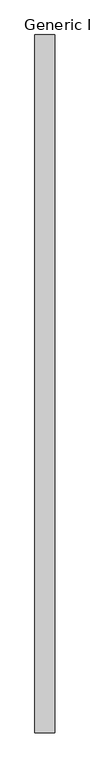
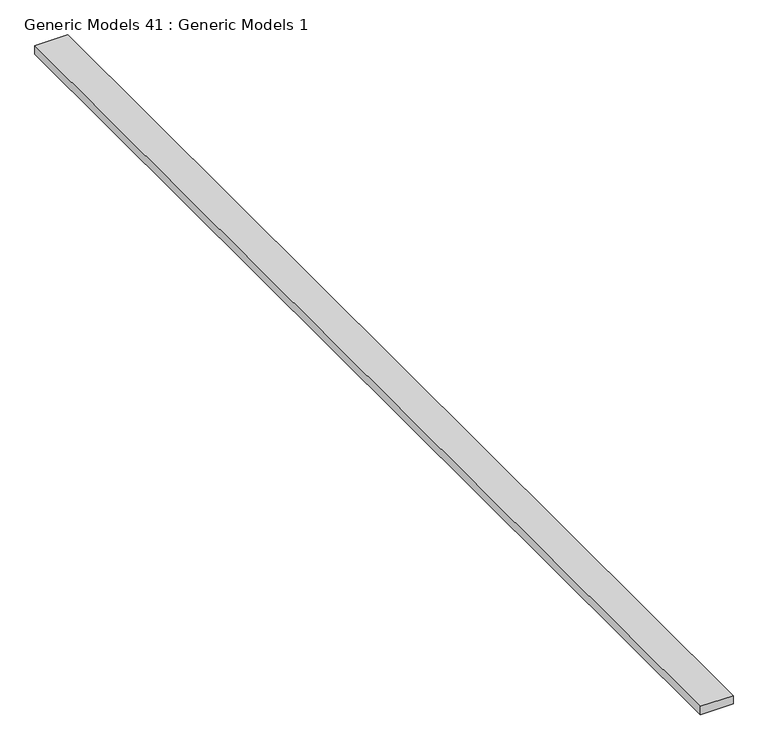
"""IFC4 building model written with IfcOpenShell, lengths in millimetres: proxy geometry, Generic Models 41 : Generic Models 1."""

from ifc_helpers import new_model, si_unit, frame, origin, place, context, project, spatial, polyline, outline, extrude, source, transform, mapped, element, save


def generic_models_41_generic_models_1_f8fef380(model_context):
    return source(origin(), model_context, "Body", "SweptSolid", [
        extrude(outline(polyline([(-9392.4319471, 11981.8769662), (-9252.7319471, 11981.8769662), (-9252.7319471, 7054.2769662), (-9392.4319471, 7054.2769662), (-9392.4319471, 11981.8769662)])), frame((0.0, 0.0, 126420.6399833), z_axis=(0.0, 0.0, 1.0), x_axis=(1.0, 0.0, 0.0)), (0.0, 0.0, 1.0), 38.1),
    ])


if __name__ == "__main__":
    model = new_model("IFC4")
    model_context = context("Model", 3, world=origin())
    ifc_project = project(units=[si_unit("LENGTHUNIT", "METRE", prefix="MILLI")], contexts=[model_context])
    site = spatial("IfcSite", under=ifc_project)
    building = spatial("IfcBuilding", under=site)
    placement = place(None, origin())
    generic_models_41_generic_models_1_shape = generic_models_41_generic_models_1_f8fef380(model_context)
    element("IfcBuildingElementProxy", 1, Name="Generic Models 41 : Generic Models 1", ObjectType="Generic Models 41 : Generic Models 1", at=placement, inside=building, context=model_context, shape_type="MappedRepresentation", body=[
        mapped(generic_models_41_generic_models_1_shape, transform((0.0, 0.0, 0.0), x_axis=(1.0, 0.0, 0.0), y_axis=(0.0, 1.0, 0.0), z_axis=(0.0, 0.0, 1.0))),
    ])
    save(model, "model.ifc")

# Revit data of these elements
# Element 1 (IfcBuildingElementProxy, "Generic Models 41 : Generic Models 1")
#   Materials on its faces: "_2X BLOCKING AS REQUIRED"
# Materials
#   "_2X BLOCKING AS REQUIRED": class "Generic", colour RGB 177 130 114, transparency 0, Cost = 0
